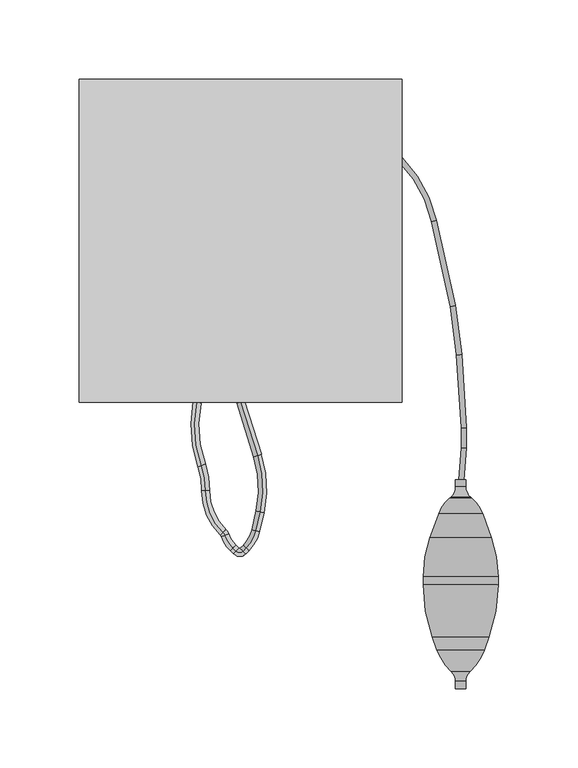
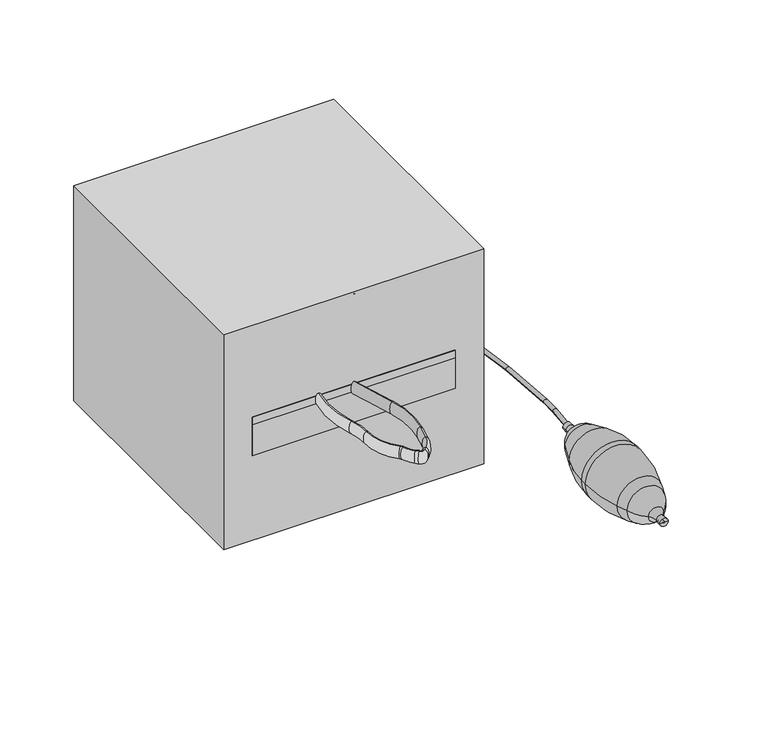
# IFC4 building model written with IfcOpenShell, lengths in millimetres: proxy geometry, M4100 - Sphygmomanometer, Aneroid, Wall-Mounted : M4100 - Sphygmomanometer, Aneroid, Wall-Mounted.
# Revit data of these elements (continued)
# Project information
#   Sheets - Total = "5"
#   Project Issue Date = "Issue Date"
#   Project Status = "Project Status"
#   Client Name = "Owner"
#   Project Address = "Enter address here"
#   Project Name = "Project Name"
#   Project Number = "Project Number"
#   Publication Date = "30-Jan-15"
# Type "M4100 - Sphygmomanometer, Aneroid, Wall-Mounted : M4100 - Sphygmomanometer, Aneroid, Wall-Mounted"
#   Watts2 = "0"
#   Watts1 = "0"
#   Unit_Issue = "EA"
#   UTIL_6_Misc = "-"
#   UTIL_5_NonMedGas = "-"
#   UTIL_4_MiscGas = "-"
#   UTIL_3_MedGas = "-"
#   UTIL_2_Elec = "-"
#   UTIL_1_WaterDrain = "-"
#   Nomenclature = "Sphygmomanometer, Aneroid, Wall Mounted"
#   NSN = "6520"
#   Location [instance default] = ""
#   JSN = "M4100"
#   Fund_Source_VA = "-"
#   Fund_Source_Navy = "-"
#   Fund_Source_Army = "-"
#   Fund_Source_AF = "-"
#   ELEC_Volts2 = "0"
#   ELEC_Volts1 = "0"
#   ELEC_Phase2 = "0"
#   ELEC_Phase1 = "0"
#   ELEC_HertzSwitch = "0"
#   ELEC_HertzDependent = "0"
#   ELEC_Hertz = "0"
#   ELEC_Amps2 = "0"
#   ELEC_Amps1 = "0"
#   DetailDescription = "Aneroid sphygmomanometer. Unit is wall mounted and has large graphic dial display for easy reading from all angles. It has a 90 degree (angle) swivel and 10 degree (angle) forward tilt to reduce glare. Unit accuracy is within 1% of reading. Sturdy impact-resistant construction."
#   CAT_VA = "C"
#   CAT_Navy = "C"
#   CAT_IHS = "-"
#   CAT_Army = "C"
#   CAT_AF = "C"
#   BTUperhour = "0"
#   mounting height [instance default] = 0' - 0"
#   Weight_IP = 5
#   Default Elevation = 4' - 0"
#   DIM_Width_IP = 0' - 8"
#   DIM_Height_IP = 0' - 8"
#   DIM_Depth_IP = 0' - 7"
#   finish [instance default] = none
#   Assembly Code = ""
# Element 1 (IfcBuildingElementProxy, "M4100 - Sphygmomanometer, Aneroid, Wall-Mounted : M4100 - Sphygmomanometer, Aneroid, Wall-Mounted")
#   Location = "TRGM1"
#   Materials on its faces: "EquipSpace"
# Materials
#   "EquipSpace": class "Unassigned", colour RGB 221 217 195, transparency 0.5
